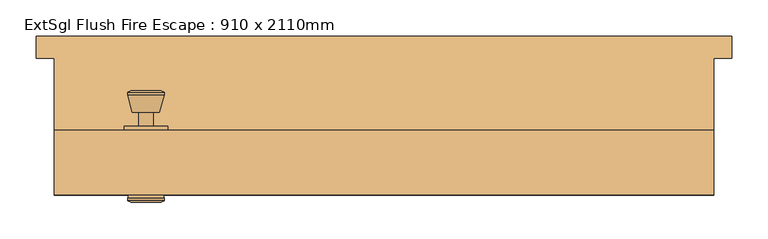
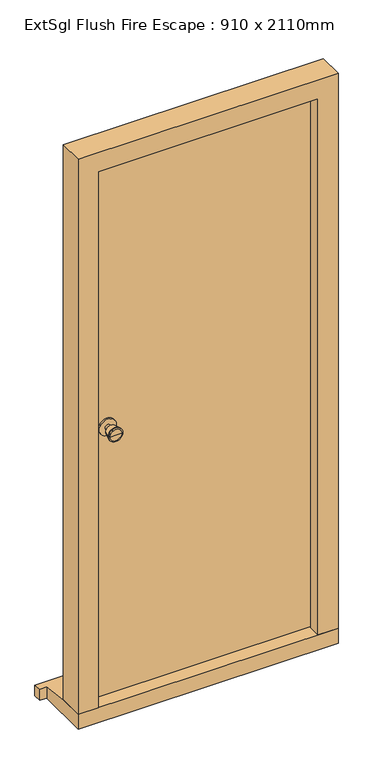
"""IFC4 building model written with IfcOpenShell, lengths in millimetres: door geometry, ExtSgl Flush Fire Escape : 910 x 2110mm."""

import ifcopenshell
import ifcopenshell.guid

model = None  # the IFC model being written
_history = None  # IfcOwnerHistory: only IFC2X3 demands one
_inside = {}  # id of a spatial element -> (the spatial element, [elements in it])
_under = {}  # id of a project, library or spatial element -> (it, [spatial elements below it])
_declared = {}  # id of a project -> (the project, [libraries it declares])
_typed = {}  # id of a type object -> (the type object, [elements of that type])
_made_of = {}  # id of a material, layer set ... -> (it, [elements and type objects made of it])


def new_model(schema):
    """Start an empty IFC model of exactly this schema.

    Asked for "IFC4X3", IfcOpenShell would pick the latest addendum, in which some entities
    have other attributes; the version numbers below select the first issue.
    IFC2X3 requires an IfcOwnerHistory on every rooted entity: one is made here for all.
    """
    global model, _history
    if schema == "IFC4X3":
        model = ifcopenshell.file(schema_version=(4, 3, 0, 0))
    else:
        model = ifcopenshell.file(schema=schema)
    _inside.clear()
    _under.clear()
    _declared.clear()
    _typed.clear()
    _made_of.clear()
    _history = None
    if model.schema == "IFC2X3":
        org = make("IfcOrganization", Name="unknown")
        user = make(
            "IfcPersonAndOrganization",
            ThePerson=make("IfcPerson", FamilyName="unknown"),
            TheOrganization=org,
        )
        app = make(
            "IfcApplication",
            ApplicationDeveloper=org,
            Version="unknown",
            ApplicationFullName="unknown",
            ApplicationIdentifier="unknown",
        )
        _history = make(
            "IfcOwnerHistory",
            OwningUser=user,
            OwningApplication=app,
            ChangeAction="ADDED",
            CreationDate=0,
        )
    return model


def make(cls, **values):
    """One entity of the class cls with the attributes given. An attribute that is None is left unset."""
    return model.create_entity(
        cls, **{name: value for name, value in values.items() if value is not None}
    )


def rooted(cls, **values):
    """An entity with a GlobalId (a new one), such as an element, a storey or a relation."""
    return make(cls, GlobalId=ifcopenshell.guid.new(), OwnerHistory=_history, **values)


def si_unit(unit_type, name, prefix=None):
    """IfcSIUnit, for example si_unit("LENGTHUNIT", "METRE", prefix="MILLI")."""
    return make("IfcSIUnit", UnitType=unit_type, Prefix=prefix, Name=name)


def assignment(units):
    """IfcUnitAssignment: the units of a project."""
    return None if units is None else make("IfcUnitAssignment", Units=units)


def point(xyz):
    """IfcCartesianPoint."""
    return None if xyz is None else make("IfcCartesianPoint", Coordinates=xyz)


def direction(xyz):
    """IfcDirection."""
    return None if xyz is None else make("IfcDirection", DirectionRatios=xyz)


def frame(location, z_axis=None, x_axis=None):
    """IfcAxis2Placement3D, a coordinate frame: its origin and axes. An axis left out is left unset."""
    return make(
        "IfcAxis2Placement3D",
        Location=point(location),
        Axis=direction(z_axis),
        RefDirection=direction(x_axis),
    )


def frame_2d(location, x_axis=None):
    """IfcAxis2Placement2D, a coordinate frame in the plane: its origin and x axis."""
    return make(
        "IfcAxis2Placement2D", Location=point(location), RefDirection=direction(x_axis)
    )


def origin():
    """The frame at (0, 0, 0) with its axes left unset."""
    return frame((0.0, 0.0, 0.0))


def place(relative_to, where):
    """IfcLocalPlacement: puts the frame where relative to a parent placement (None: the world)."""
    return make(
        "IfcLocalPlacement", PlacementRelTo=relative_to, RelativePlacement=where
    )


def context(
    kind, dimensions, precision=None, world=None, true_north=None, identifier=None
):
    """IfcGeometricRepresentationContext, for example the 3D "Model" context."""
    return make(
        "IfcGeometricRepresentationContext",
        ContextIdentifier=identifier,
        ContextType=kind,
        CoordinateSpaceDimension=dimensions,
        Precision=precision,
        WorldCoordinateSystem=world,
        TrueNorth=true_north,
    )


def project(units=None, contexts=None):
    """IfcProject with its units and contexts."""
    return rooted(
        "IfcProject",
        Name="project",
        RepresentationContexts=contexts,
        UnitsInContext=assignment(units),
    )


def spatial(cls, under=None, at=None, **own):
    """A site, building, storey or space (cls), placed at a placement, below another one or the project."""
    s = rooted(cls, ObjectPlacement=at, **own)
    if under is not None:
        _under.setdefault(under.id(), (under, []))[1].append(s)
    return s


def polyline(points):
    """IfcPolyline through the points."""
    return make("IfcPolyline", Points=[point(p) for p in points])


def circle_curve(where, radius):
    """IfcCircle in the frame where."""
    return make("IfcCircle", Position=where, Radius=radius)


def trimmed(basis, trim1, trim2, sense, master):
    """IfcTrimmedCurve: the piece of a basis curve between two trims."""
    return make(
        "IfcTrimmedCurve",
        BasisCurve=basis,
        Trim1=trim1,
        Trim2=trim2,
        SenseAgreement=sense,
        MasterRepresentation=master,
    )


def segment(curve, same_sense, transition):
    """IfcCompositeCurveSegment."""
    return make(
        "IfcCompositeCurveSegment",
        Transition=transition,
        SameSense=same_sense,
        ParentCurve=curve,
    )


def composite_curve(segments, self_intersect=None):
    """IfcCompositeCurve: segments joined end to end."""
    return make("IfcCompositeCurve", Segments=segments, SelfIntersect=self_intersect)


def outline(outer, holes=None, kind="AREA"):
    """IfcArbitraryClosedProfileDef: a profile drawn as a closed curve; with holes, ...WithVoids."""
    if holes is None:
        return make("IfcArbitraryClosedProfileDef", ProfileType=kind, OuterCurve=outer)
    return make(
        "IfcArbitraryProfileDefWithVoids",
        ProfileType=kind,
        OuterCurve=outer,
        InnerCurves=holes,
    )


def extrude(swept, where, along, depth):
    """IfcExtrudedAreaSolid: the profile swept, set in the frame where, extruded along a direction by depth."""
    return make(
        "IfcExtrudedAreaSolid",
        SweptArea=swept,
        Position=where,
        ExtrudedDirection=direction(along),
        Depth=depth,
    )


def faces_of(points, faces, orient=None, outer=None):
    """IfcFace entities. A face is a list of loops; a loop is a list of indices into points, from 0.

    orient and outer hold one flag for each loop. By default every Orientation is true, the
    first loop of a face is its IfcFaceOuterBound and the others are IfcFaceBound.
    """
    made = []
    for i, loops in enumerate(faces):
        bounds = []
        for j, loop in enumerate(loops):
            is_outer = j == 0 if outer is None else outer[i][j]
            bounds.append(
                make(
                    "IfcFaceOuterBound" if is_outer else "IfcFaceBound",
                    Bound=make("IfcPolyLoop", Polygon=[points[k] for k in loop]),
                    Orientation=True if orient is None else orient[i][j],
                )
            )
        made.append(make("IfcFace", Bounds=bounds))
    return made


def faceted_brep(points, faces, orient=None, outer=None, voids=None):
    """IfcFacetedBrep: a solid bounded by flat faces; with voids (closed shells), ...WithVoids."""
    shared = [point(p) for p in points]
    hull = make("IfcClosedShell", CfsFaces=faces_of(shared, faces, orient, outer))
    if voids is None:
        return make("IfcFacetedBrep", Outer=hull)
    return make(
        "IfcFacetedBrepWithVoids",
        Outer=hull,
        Voids=[
            make(cls, CfsFaces=faces_of(shared, fs, o, b)) for cls, fs, o, b in voids
        ],
    )


def shape(context_of_items, identifier, shape_type, items):
    """IfcShapeRepresentation: the items that make up one representation, for example the "Body"."""
    return make(
        "IfcShapeRepresentation",
        ContextOfItems=context_of_items,
        RepresentationIdentifier=identifier,
        RepresentationType=shape_type,
        Items=items,
    )


def source(mapping_origin, context_of_items, identifier, shape_type, items):
    """IfcRepresentationMap: a shape defined once, which mapped items show again and again."""
    return make(
        "IfcRepresentationMap",
        MappingOrigin=mapping_origin,
        MappedRepresentation=shape(context_of_items, identifier, shape_type, items),
    )


def transform(
    local_origin,
    x_axis=None,
    y_axis=None,
    z_axis=None,
    scale=None,
    scale2=None,
    scale3=None,
    uniform=True,
):
    """IfcCartesianTransformationOperator3D, or its non-uniform kind. x_axis, y_axis, z_axis: its Axis1, 2, 3."""
    if uniform:
        return make(
            "IfcCartesianTransformationOperator3D",
            Axis1=direction(x_axis),
            Axis2=direction(y_axis),
            LocalOrigin=point(local_origin),
            Scale=scale,
            Axis3=direction(z_axis),
        )
    return make(
        "IfcCartesianTransformationOperator3DnonUniform",
        Axis1=direction(x_axis),
        Axis2=direction(y_axis),
        LocalOrigin=point(local_origin),
        Scale=scale,
        Axis3=direction(z_axis),
        Scale2=scale2,
        Scale3=scale3,
    )


def mapped(mapping_source, mapping_target):
    """IfcMappedItem: shows the shape of a source again, moved by a transform."""
    return make(
        "IfcMappedItem", MappingSource=mapping_source, MappingTarget=mapping_target
    )


def made_of(thing, what):
    """Note that an element or type object is made of a material, layer set ...; save() writes the relation."""
    if what is not None:
        _made_of.setdefault(what.id(), (what, []))[1].append(thing)
    return thing


def element(
    cls,
    number,
    at=None,
    inside=None,
    cuts=None,
    type_object=None,
    material=None,
    context=None,
    identifier="Body",
    shape_type=None,
    held_by="IfcProductDefinitionShape",
    body=None,
    shapes=None,
    **own,
):
    """One element of the class cls, such as IfcWall. Its Tag is "e" and its number.

    at: its placement. inside: the storey or other place that contains it. cuts: it is an
    opening in that element (IfcRelVoidsElement). A single representation is given by context,
    identifier, shape_type and body (its items); several are given by shapes. held_by: the class
    of the entity that holds the representations. save() writes the other relations.
    """
    e = rooted(cls, Tag="e%d" % number, ObjectPlacement=at, **own)
    if body is not None:
        shapes = [shape(context, identifier, shape_type, body)]
    if shapes is not None:
        e.Representation = make(held_by, Representations=shapes)
    if inside is not None:
        _inside.setdefault(inside.id(), (inside, []))[1].append(e)
    if cuts is not None:
        rooted(
            "IfcRelVoidsElement", RelatingBuildingElement=cuts, RelatedOpeningElement=e
        )
    if type_object is not None:
        _typed.setdefault(type_object.id(), (type_object, []))[1].append(e)
    return made_of(e, material)


def aggregate(whole, parts):
    """IfcRelAggregates: a whole, such as a stair, and the parts it consists of."""
    return rooted("IfcRelAggregates", RelatingObject=whole, RelatedObjects=parts)


def save(model, path):
    """Write the relations noted so far, then the file.

    IfcRelAggregates (storeys below a building ...), IfcRelContainedInSpatialStructure (elements
    in a storey), IfcRelDefinesByType, IfcRelAssociatesMaterial and IfcRelDeclares: one each for
    every whole, place, type object, material and project.
    """
    for whole, parts in _under.values():
        aggregate(whole, parts)
    for where, things in _inside.values():
        rooted(
            "IfcRelContainedInSpatialStructure",
            RelatedElements=things,
            RelatingStructure=where,
        )
    for kind, things in _typed.values():
        rooted("IfcRelDefinesByType", RelatedObjects=things, RelatingType=kind)
    for what, things in _made_of.values():
        rooted("IfcRelAssociatesMaterial", RelatedObjects=things, RelatingMaterial=what)
    for by, libraries in _declared.values():
        rooted("IfcRelDeclares", RelatingContext=by, RelatedDefinitions=libraries)
    model.write(path)


def plane_surface(at):
    """IfcPlane: the flat surface through the origin of the frame at, square to its z axis."""
    return make("IfcPlane", Position=at)


def cylinder_surface(at, radius):
    """IfcCylindricalSurface: all points at the distance radius from the z axis of the frame at."""
    return make("IfcCylindricalSurface", Position=at, Radius=radius)


def revolved_surface(curve, axis_point, axis_direction):
    """IfcSurfaceOfRevolution: the curve turned about the line through axis_point along axis_direction."""
    return make(
        "IfcSurfaceOfRevolution",
        SweptCurve=make("IfcArbitraryOpenProfileDef", ProfileType="CURVE", Curve=curve),
        AxisPosition=make("IfcAxis1Placement", Location=point(axis_point), Axis=direction(axis_direction)),
    )


def advanced_brep(points, edges, surfaces, faces):
    """IfcAdvancedBrep: a solid bounded by faces that lie on surfaces and meet in shared edges.

    An edge is (start, end): straight between two places in points (the first is 0);
    or (start, end, curve); or (start, end, curve, False) where it runs against its curve.
    A face is (place in surfaces, loops), or (place, loops, False) where it looks against
    its surface's normal. A loop lists edges by number (the first is 1), with a minus sign
    where the edge is run from its end to its start. The first loop is the outer one.
    """
    corners = [point(p) for p in points]
    vertices = [make("IfcVertexPoint", VertexGeometry=c) for c in corners]
    made = []
    for start, end, *more in edges:
        made.append(
            make(
                "IfcEdgeCurve",
                EdgeStart=vertices[start],
                EdgeEnd=vertices[end],
                EdgeGeometry=more[0] if more else make("IfcPolyline", Points=[corners[start], corners[end]]),
                SameSense=more[1] if len(more) > 1 else True,
            )
        )
    hull = []
    for where, loops, *sense in faces:
        bounds = []
        for j, loop in enumerate(loops):
            ring = [make("IfcOrientedEdge", EdgeElement=made[abs(k) - 1], Orientation=k > 0) for k in loop]
            bounds.append(
                make(
                    "IfcFaceOuterBound" if j == 0 else "IfcFaceBound",
                    Bound=make("IfcEdgeLoop", EdgeList=ring),
                    Orientation=True,
                )
            )
        hull.append(make("IfcAdvancedFace", Bounds=bounds, FaceSurface=surfaces[where], SameSense=sense[0] if sense else True))
    return make("IfcAdvancedBrep", Outer=make("IfcClosedShell", CfsFaces=hull))


def extsgl_flush_fire_escape_910_x_2110mm_612fc41a(model_context):
    return source(origin(), model_context, "Body", "SolidModel", [
        advanced_brep(
        [(-328.5, 121.0, 1050.0), (-338.5, 121.0, 1050.0), (-318.5, 121.0, 1050.0), (-308.0241324, 170.0, 1050.0), (-348.9758676, 170.0, 1050.0), (-328.5, 170.0, 1050.0), (-303.5, 168.1721319, 1050.0), (-353.5, 168.1721319, 1050.0), (-303.5, 164.7084537, 1050.0), (-353.5, 164.7084537, 1050.0), (-309.863764, 140.0, 1050.0), (-347.136236, 140.0, 1050.0), (-318.5, 140.0, 1050.0), (-338.5, 140.0, 1050.0)],
        [
            (0, 1),
            (1, 2, circle_curve(frame((-328.5, 121.0, 1050.0), z_axis=(0.0, -1.0, 0.0), x_axis=(-1.0, 0.0, 0.0)), 10.0)),
            (2, 0),
            (2, 1, circle_curve(frame((-328.5, 121.0, 1050.0), z_axis=(0.0, -1.0, 0.0), x_axis=(-1.0, 0.0, 0.0)), 10.0)),
            (3, 4, circle_curve(frame((-328.5, 170.0, 1050.0), z_axis=(0.0, 1.0, 0.0), x_axis=(-1.0, 0.0, 0.0)), 20.4758676)),
            (4, 5),
            (5, 3),
            (4, 3, circle_curve(frame((-328.5, 170.0, 1050.0), z_axis=(0.0, 1.0, 0.0), x_axis=(-1.0, 0.0, 0.0)), 20.4758676)),
            (6, 7, circle_curve(frame((-328.5, 168.1721319, 1050.0), z_axis=(0.0, 1.0, 0.0), x_axis=(-1.0, 0.0, 0.0)), 25.0)),
            (7, 4),
            (3, 6),
            (7, 6, circle_curve(frame((-328.5, 168.1721319, 1050.0), z_axis=(0.0, 1.0, 0.0), x_axis=(-1.0, 0.0, 0.0)), 25.0)),
            (8, 9, circle_curve(frame((-328.5, 164.7084537, 1050.0), z_axis=(0.0, 1.0, 0.0), x_axis=(-1.0, 0.0, 0.0)), 25.0)),
            (9, 7),
            (6, 8),
            (9, 8, circle_curve(frame((-328.5, 164.7084537, 1050.0), z_axis=(0.0, 1.0, 0.0), x_axis=(-1.0, 0.0, 0.0)), 25.0)),
            (10, 11, circle_curve(frame((-328.5, 140.0, 1050.0), z_axis=(0.0, 1.0, 0.0), x_axis=(-1.0, 0.0, 0.0)), 18.636236)),
            (11, 9),
            (8, 10),
            (11, 10, circle_curve(frame((-328.5, 140.0, 1050.0), z_axis=(0.0, 1.0, 0.0), x_axis=(-1.0, 0.0, 0.0)), 18.636236)),
            (12, 13, circle_curve(frame((-328.5, 140.0, 1050.0), z_axis=(0.0, 1.0, 0.0), x_axis=(-1.0, 0.0, 0.0)), 10.0)),
            (13, 11),
            (10, 12),
            (13, 12, circle_curve(frame((-328.5, 140.0, 1050.0), z_axis=(0.0, 1.0, 0.0), x_axis=(-1.0, 0.0, 0.0)), 10.0)),
            (1, 13),
            (12, 2),
        ],
        [
            plane_surface(frame((-328.5, 121.0, 1050.0), z_axis=(0.0, -1.0, 0.0), x_axis=(-1.0, 0.0, 0.0))),
            plane_surface(frame((-328.5, 170.0, 1050.0), z_axis=(0.0, 1.0, 0.0), x_axis=(-1.0, 0.0, 0.0))),
            revolved_surface(polyline([(-348.9758676, 170.0, 1050.0), (-353.5, 168.1721319, 1050.0)]), (-328.5, 121.0, 1050.0), (0.0, -1.0, 0.0)),
            cylinder_surface(frame((-328.5, 121.0, 1050.0), z_axis=(0.0, -1.0, 0.0), x_axis=(-1.0, 0.0, 0.0)), 25.0),
            revolved_surface(polyline([(-353.5, 164.7084537, 1050.0), (-347.136236, 140.0, 1050.0)]), (-328.5, 121.0, 1050.0), (0.0, -1.0, 0.0)),
            plane_surface(frame((-328.5, 140.0, 1050.0), z_axis=(0.0, -1.0, 0.0), x_axis=(-1.0, 0.0, 0.0))),
            cylinder_surface(frame((-328.5, 121.0, 1050.0), z_axis=(0.0, -1.0, 0.0), x_axis=(-1.0, 0.0, 0.0)), 10.0),
        ],
        [
            (0, [[1, 2, 3]]),
            (0, [[-3, 4, -1]]),
            (1, [[5, 6, 7]]),
            (1, [[8, -7, -6]]),
            (2, [[9, 10, -5, 11]]),
            (2, [[12, -11, -8, -10]]),
            (3, [[13, 14, -9, 15]]),
            (3, [[16, -15, -12, -14]]),
            (4, [[17, 18, -13, 19]]),
            (4, [[20, -19, -16, -18]]),
            (5, [[21, 22, -17, 23]]),
            (5, [[24, -23, -20, -22]]),
            (6, [[-2, 25, -21, 26]]),
            (6, [[-4, -26, -24, -25]]),
        ],
    ),
        extrude(outline(composite_curve([segment(trimmed(circle_curve(frame_2d((1050.0, -328.5)), 30.0), [point((1050.0, -358.5))], [point((1050.0, -298.5))], False, "CARTESIAN"), True, "CONTINUOUS"), segment(trimmed(circle_curve(frame_2d((1050.0, -328.5)), 30.0), [point((1050.0, -298.5))], [point((1050.0, -358.5))], False, "CARTESIAN"), True, "CONTINUOUS")], self_intersect=False)), frame((0.0, 115.0, 0.0), z_axis=(0.0, 1.0, 0.0), x_axis=(0.0, 0.0, 1.0)), (0.0, 0.0, 1.0), 6.0),
        advanced_brep(
        [(-328.5, 65.0, 1050.0), (-318.5, 65.0, 1050.0), (-338.5, 65.0, 1050.0), (-308.0241324, 16.0, 1050.0), (-328.5, 16.0, 1050.0), (-348.9758676, 16.0, 1050.0), (-303.5, 17.8278681, 1050.0), (-353.5, 17.8278681, 1050.0), (-303.5, 21.2915463, 1050.0), (-353.5, 21.2915463, 1050.0), (-309.863764, 46.0, 1050.0), (-347.136236, 46.0, 1050.0), (-318.5, 46.0, 1050.0), (-338.5, 46.0, 1050.0)],
        [
            (0, 1),
            (1, 2, circle_curve(frame((-328.5, 65.0, 1050.0), z_axis=(0.0, 1.0, 0.0), x_axis=(-1.0, 0.0, 0.0)), 10.0)),
            (2, 0),
            (2, 1, circle_curve(frame((-328.5, 65.0, 1050.0), z_axis=(0.0, 1.0, 0.0), x_axis=(-1.0, 0.0, 0.0)), 10.0)),
            (3, 4),
            (4, 5),
            (5, 3, circle_curve(frame((-328.5, 16.0, 1050.0), z_axis=(0.0, -1.0, 0.0), x_axis=(-1.0, 0.0, 0.0)), 20.4758676)),
            (3, 5, circle_curve(frame((-328.5, 16.0, 1050.0), z_axis=(0.0, -1.0, 0.0), x_axis=(-1.0, 0.0, 0.0)), 20.4758676)),
            (6, 3),
            (5, 7),
            (7, 6, circle_curve(frame((-328.5, 17.8278681, 1050.0), z_axis=(0.0, -1.0, 0.0), x_axis=(-1.0, 0.0, 0.0)), 25.0)),
            (6, 7, circle_curve(frame((-328.5, 17.8278681, 1050.0), z_axis=(0.0, -1.0, 0.0), x_axis=(-1.0, 0.0, 0.0)), 25.0)),
            (8, 6),
            (7, 9),
            (9, 8, circle_curve(frame((-328.5, 21.2915463, 1050.0), z_axis=(0.0, -1.0, 0.0), x_axis=(-1.0, 0.0, 0.0)), 25.0)),
            (8, 9, circle_curve(frame((-328.5, 21.2915463, 1050.0), z_axis=(0.0, -1.0, 0.0), x_axis=(-1.0, 0.0, 0.0)), 25.0)),
            (10, 8),
            (9, 11),
            (11, 10, circle_curve(frame((-328.5, 46.0, 1050.0), z_axis=(0.0, -1.0, 0.0), x_axis=(-1.0, 0.0, 0.0)), 18.636236)),
            (10, 11, circle_curve(frame((-328.5, 46.0, 1050.0), z_axis=(0.0, -1.0, 0.0), x_axis=(-1.0, 0.0, 0.0)), 18.636236)),
            (12, 10),
            (11, 13),
            (13, 12, circle_curve(frame((-328.5, 46.0, 1050.0), z_axis=(0.0, -1.0, 0.0), x_axis=(-1.0, 0.0, 0.0)), 10.0)),
            (12, 13, circle_curve(frame((-328.5, 46.0, 1050.0), z_axis=(0.0, -1.0, 0.0), x_axis=(-1.0, 0.0, 0.0)), 10.0)),
            (1, 12),
            (13, 2),
        ],
        [
            plane_surface(frame((-328.5, 65.0, 1050.0), z_axis=(0.0, 1.0, 0.0), x_axis=(-1.0, 0.0, 0.0))),
            plane_surface(frame((-328.5, 16.0, 1050.0), z_axis=(0.0, -1.0, 0.0), x_axis=(-1.0, 0.0, 0.0))),
            revolved_surface(polyline([(-348.9758676, 16.0, 1050.0), (-353.5, 17.8278681, 1050.0)]), (-328.5, 65.0, 1050.0), (0.0, 1.0, 0.0)),
            cylinder_surface(frame((-328.5, 65.0, 1050.0), z_axis=(0.0, 1.0, 0.0), x_axis=(-1.0, 0.0, 0.0)), 25.0),
            revolved_surface(polyline([(-353.5, 21.2915463, 1050.0), (-347.136236, 46.0, 1050.0)]), (-328.5, 65.0, 1050.0), (0.0, 1.0, 0.0)),
            plane_surface(frame((-328.5, 46.0, 1050.0), z_axis=(0.0, 1.0, 0.0), x_axis=(-1.0, 0.0, 0.0))),
            cylinder_surface(frame((-328.5, 65.0, 1050.0), z_axis=(0.0, 1.0, 0.0), x_axis=(-1.0, 0.0, 0.0)), 10.0),
        ],
        [
            (0, [[1, 2, 3]]),
            (0, [[-3, 4, -1]]),
            (1, [[5, 6, 7]]),
            (1, [[-6, -5, 8]]),
            (2, [[9, -7, 10, 11]]),
            (2, [[-10, -8, -9, 12]]),
            (3, [[13, -11, 14, 15]]),
            (3, [[-14, -12, -13, 16]]),
            (4, [[17, -15, 18, 19]]),
            (4, [[-18, -16, -17, 20]]),
            (5, [[21, -19, 22, 23]]),
            (5, [[-22, -20, -21, 24]]),
            (6, [[25, -23, 26, -2]]),
            (6, [[-26, -24, -25, -4]]),
        ],
    ),
        extrude(outline(composite_curve([segment(trimmed(circle_curve(frame_2d((1050.0, -328.5)), 30.0), [point((1050.0, -358.5))], [point((1050.0, -298.5))], False, "CARTESIAN"), True, "CONTINUOUS"), segment(trimmed(circle_curve(frame_2d((1050.0, -328.5)), 30.0), [point((1050.0, -298.5))], [point((1050.0, -358.5))], False, "CARTESIAN"), True, "CONTINUOUS")], self_intersect=False)), frame((0.0, 65.0, 0.0), z_axis=(0.0, 1.0, 0.0), x_axis=(0.0, 0.0, 1.0)), (0.0, 0.0, 1.0), 6.0),
        faceted_brep([(406.5, 115.0, 54.5), (455.0, 115.0, 54.5), (455.0, 26.0, 54.5), (384.5, 26.0, 54.5), (384.5, 68.0, 54.5), (406.5, 68.0, 54.5), (406.5, 115.0, 2061.5), (-406.5, 115.0, 2061.5), (-406.5, 115.0, 54.5), (-455.0, 115.0, 54.5), (-455.0, 115.0, 2110.0), (455.0, 115.0, 2110.0), (455.0, 26.0, 2110.0), (-455.0, 26.0, 2110.0), (-455.0, 26.0, 54.5), (-384.5, 26.0, 54.5), (-384.5, 26.0, 2039.5), (384.5, 26.0, 2039.5), (384.5, 68.0, 2039.5), (-384.5, 68.0, 2039.5), (-384.5, 68.0, 54.5), (-406.5, 68.0, 54.5), (-406.5, 68.0, 2061.5), (406.5, 68.0, 2061.5)], [[[0, 1, 2, 3, 4, 5]], [[1, 0, 6, 7, 8, 9, 10, 11]], [[2, 1, 11, 12]], [[3, 2, 12, 13, 14, 15, 16, 17]], [[4, 3, 17, 18]], [[5, 4, 18, 19, 20, 21, 22, 23]], [[0, 5, 23, 6]], [[7, 22, 21, 8]], [[8, 21, 20, 15, 14, 9]], [[13, 10, 9, 14]], [[19, 16, 15, 20]], [[12, 11, 10, 13]], [[18, 17, 16, 19]], [[6, 23, 22, 7]]]),
        faceted_brep([(480.0, 245.0, 0.0), (480.0, 245.0, 38.5947221), (480.0, 215.0, 42.2651709), (480.0, 215.0, 0.0), (-480.0, 245.0, 38.5947221), (-480.0, 245.0, 0.0), (-480.0, 215.0, 0.0), (-480.0, 215.0, 42.2651709), (455.0, 215.0, 0.0), (455.0, 26.0, 0.0), (-455.0, 26.0, 0.0), (-455.0, 215.0, 0.0), (-455.0, 215.0, 42.2651709), (-455.0, 115.0, 54.5), (455.0, 115.0, 54.5), (455.0, 215.0, 42.2651709), (-455.0, 26.0, 54.5), (455.0, 26.0, 54.5)], [[[0, 1, 2, 3]], [[4, 5, 6, 7]], [[5, 0, 3, 8, 9, 10, 11, 6]], [[1, 0, 5, 4]], [[1, 4, 7, 12, 13, 14, 15, 2]], [[13, 16, 17, 14]], [[16, 10, 9, 17]], [[12, 11, 10, 16, 13]], [[11, 12, 7, 6]], [[8, 15, 14, 17, 9]], [[15, 8, 3, 2]]]),
        extrude(outline(polyline([(403.5, 71.0), (-404.4250294, 71.0), (-404.4250294, 115.0), (403.5, 115.0), (403.5, 71.0)])), frame((0.0, 0.0, 58.5), z_axis=(0.0, 0.0, 1.0), x_axis=(1.0, 0.0, 0.0)), (0.0, 0.0, 1.0), 2000.0),
    ])


if __name__ == "__main__":
    model = new_model("IFC4")
    model_context = context("Model", 3, world=origin())
    ifc_project = project(units=[si_unit("LENGTHUNIT", "METRE", prefix="MILLI")], contexts=[model_context])
    site = spatial("IfcSite", under=ifc_project)
    building = spatial("IfcBuilding", under=site)
    placement = place(None, origin())
    extsgl_flush_fire_escape_910_x_2110mm_shape = extsgl_flush_fire_escape_910_x_2110mm_612fc41a(model_context)
    element("IfcDoor", 1, ObjectType="ExtSgl Flush Fire Escape : 910 x 2110mm", at=placement, inside=building, context=model_context, shape_type="MappedRepresentation", body=[
        mapped(extsgl_flush_fire_escape_910_x_2110mm_shape, transform((0.0, 0.0, 0.0), x_axis=(1.0, 0.0, 0.0), y_axis=(0.0, 1.0, 0.0), z_axis=(0.0, 0.0, 1.0))),
    ])
    save(model, "model.ifc")

# Revit data of these elements
# Type "ExtSgl Flush Fire Escape : 910 x 2110mm"
#   Description = "Fire Escape Door"
#   Type Mark = "57"
#   Type Comments = "External Single"
#   Operation = "SingleSwingRight"
#   Construction Type Id = "MDOOR"
#   Keynote = "L20"
#   Analytic Construction = "Metal"
#   Wrap Layers (Int) from Ext = 177.5 mm
#   Wrap Layers (Ext) from Ext = 102.5 mm
#   Thickness = 44 mm
#   Rough Width = 910 mm
#   Rough Height = 2110 mm
#   O/A Frame Width = 64 mm
#   Heat Transfer Coefficient (U) = 3.7021 W/(m²·K)
#   Handle Z Distance = 1050 mm
#   FrameWidth = 42 mm
#   FrameOffset - External = 100 mm
#   FrameDepth = 89 mm
#   Door Panel Width = 807 mm
#   Door Panel Thickness = 44 mm
#   Door Panel Height = 2000 mm
#   Cill Thickness = 54.5 mm
#   Cill Projection = 30 mm
#   Handle X Distance = 75 mm
#   Height = 2110 mm
#   Structural Tolerance = 6.5 mm
#   Tolerance = 3 mm
#   Undercut = 4 mm
#   Width = 910 mm
#   Cill Extension = 25 mm
#   Cavity Closer Width = 75 mm
#   Cavity Closer Offset from Ext = 120 mm
#   Cavity Closer Depth = 95 mm
#   Vis - Ironmongery = yes
#   Vis - Cavity Closers = yes
#   Define Thermal Properties by = 1
#   Function = 1
#   Material Door = Door - Panel
#   Material Frame = Door - Frame/Mullion
#   Material Ironmongery = Door - Handle
#   Visual Light Transmittance = 0
#   Solar Heat Gain Coefficient = 0
#   Wall Closure = (empty or 0)
# Element 1 (IfcDoor, "ExtSgl Flush Fire Escape : 910 x 2110mm")
#   Materials on its faces: "Door - Handle", "Door - Frame/Mullion", "Door - Panel"
# Materials
#   "Door - Panel": class "Wood", colour RGB 210 159 95, transparency 0, Keynote = "L20"
#   "Door - Frame/Mullion": class "Wood", colour RGB 212 179 113, transparency 0, Keynote = "L20"
#   "Door - Handle": class "Miscellaneous", colour RGB 0 0 0, transparency 0, Keynote = "P21"
